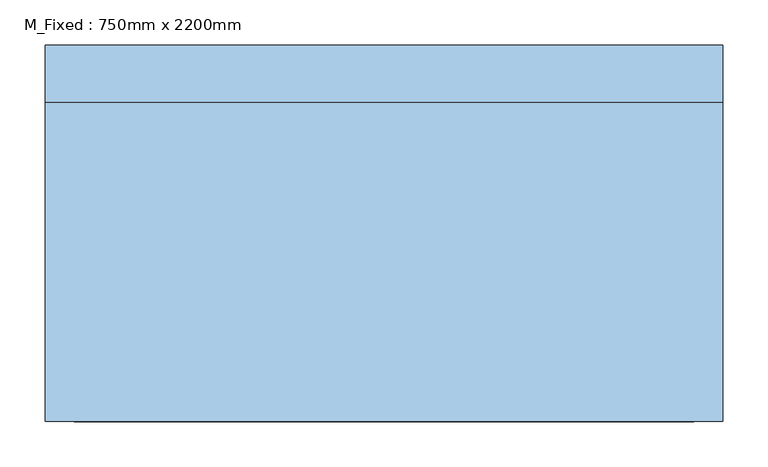
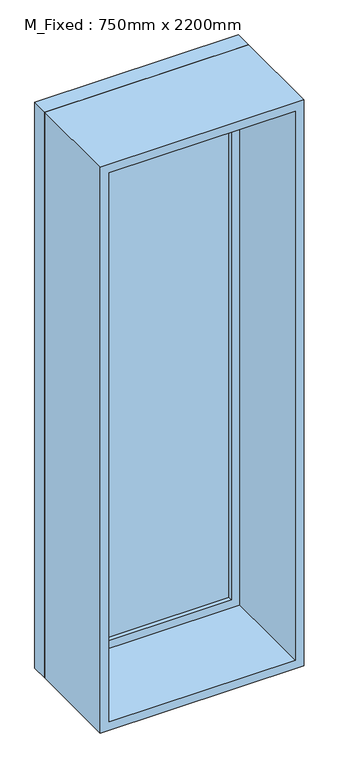
"""IFC4 building model written with IfcOpenShell, lengths in millimetres: window geometry, M_Fixed : 750mm x 2200mm."""

from ifc_helpers import new_model, si_unit, frame, origin, place, context, project, spatial, polyline, outline, extrude, source, transform, mapped, element, save


def m_fixed_750mm_x_2200mm_8ca0da28(model_context):
    return source(origin(), model_context, "Body", "SweptSolid", [
        extrude(outline(polyline([(-312.0, 186.5), (312.0, 186.5), (312.0, 174.5), (-312.0, 174.5), (-312.0, 186.5)])), frame((0.0, 0.0, 163.0), z_axis=(0.0, 0.0, 1.0), x_axis=(1.0, 0.0, 0.0)), (0.0, 0.0, 1.0), 2074.0),
        extrude(outline(polyline([(2281.0, -356.0), (119.0, -356.0), (119.0, 356.0), (2281.0, 356.0), (2281.0, -356.0)]), holes=[polyline([(2237.0, -312.0), (2237.0, 312.0), (163.0, 312.0), (163.0, -312.0), (2237.0, -312.0)])]), frame((0.0, 158.5, 0.0), z_axis=(0.0, 1.0, 0.0), x_axis=(0.0, 0.0, 1.0)), (0.0, 0.0, 1.0), 44.0),
        extrude(outline(polyline([(2300.0, -375.0), (100.0, -375.0), (100.0, 375.0), (2300.0, 375.0), (2300.0, -375.0)]), holes=[polyline([(2281.0, -356.0), (2281.0, 356.0), (119.0, 356.0), (119.0, -356.0), (2281.0, -356.0)])]), frame((0.0, 158.5, 0.0), z_axis=(0.0, 1.0, 0.0), x_axis=(0.0, 0.0, 1.0)), (0.0, 0.0, 1.0), 63.0),
        extrude(outline(polyline([(2300.0, -375.0), (100.0, -375.0), (100.0, 375.0), (2300.0, 375.0), (2300.0, -375.0)]), holes=[polyline([(2268.0, -343.0), (2268.0, 343.0), (132.0, 343.0), (132.0, -343.0), (2268.0, -343.0)])]), frame((0.0, -195.5, 0.0), z_axis=(0.0, 1.0, 0.0), x_axis=(0.0, 0.0, 1.0)), (0.0, 0.0, 1.0), 354.0),
    ])


if __name__ == "__main__":
    model = new_model("IFC4")
    model_context = context("Model", 3, world=origin())
    ifc_project = project(units=[si_unit("LENGTHUNIT", "METRE", prefix="MILLI")], contexts=[model_context])
    site = spatial("IfcSite", under=ifc_project)
    building = spatial("IfcBuilding", under=site)
    placement = place(None, origin())
    m_fixed_750mm_x_2200mm_shape = m_fixed_750mm_x_2200mm_8ca0da28(model_context)
    element("IfcWindow", 1, ObjectType="M_Fixed : 750mm x 2200mm", at=placement, inside=building, context=model_context, shape_type="MappedRepresentation", body=[
        mapped(m_fixed_750mm_x_2200mm_shape, transform((0.0, 0.0, 0.0), x_axis=(1.0, 0.0, 0.0), y_axis=(0.0, 1.0, 0.0), z_axis=(0.0, 0.0, 1.0))),
    ])
    save(model, "model.ifc")

# Revit data of these elements
# Type "M_Fixed : 750mm x 2200mm"
#   Manufacturer = "Manufacturer"
#   Type Mark = "04"
#   Construction Type = "Construction Type"
#   AccessibilityPerformance = "AccessibilityPerformance"
#   CodePerformance = "CodePerformance"
#   ConfigurationType = "ConfigurationType"
#   ConstructionType = "ConstructionType"
#   FireRating = "FireRating"
#   GlazingAreaFraction = "GlazingAreaFraction"
#   OperationType = "OperationType"
#   Area = "Area"
#   Color = "Color"
#   Constituents = "Constituents"
#   Features = "Features"
#   Finish = "Finish"
#   Grade = "Grade"
#   Material = "Material"
#   ModelReference = "ModelReference"
#   NominalHeight = "NominalHeight"
#   NominalLength = "NominalLength"
#   NominalWidth = "NominalWidth"
#   ProductionYear = "ProductionYear"
#   Reference = "Reference"
#   Shape = "Shape"
#   Size = "Size"
#   SustainabilityPerformance = "SustainabilityPerformance"
#   WarrantyDescription = "WarrantyDescription"
#   WarrantyDurationLabor = "WarrantyDurationLabor"
#   WarrantyDurationParts = "WarrantyDurationParts"
#   WarrantyGuarantorLabor = "WarrantyGuarantorLabor"
#   WarrantyGuarantorParts = "WarrantyGuarantorParts"
#   ExpectedLife = "ExpectedLife"
#   ReplacementCost = "ReplacementCost"
#   AssetAccountingType = "FIXED"
#   ModelLabel = "ModelLabel"
#   Height = 2.200 m
#   Default Sill Height = 0.100 m
#   Width = 0.750 m
#   Window Inset = 0.019 m
#   Frame Exterior Material = Sash
#   Frame Interior Material = Sash
#   Glass Pane Material = Glass
#   Sash = Sash
#   Wall Closure = (empty or 0)
# Element 1 (IfcWindow, "M_Fixed : 750mm x 2200mm")
#   Materials on its faces: "Sash", "Glass"
# Materials
#   "Sash": class "Wood", colour RGB 224 178 126, transparency 0
#   "Glass": class "Glass", colour RGB 0 128 192, transparency 0.9
